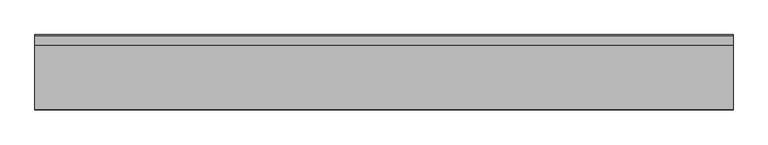
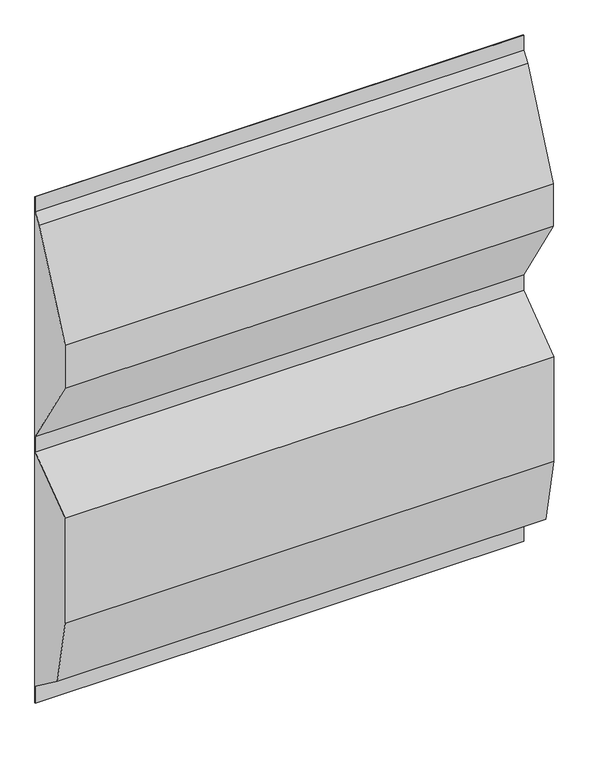
"""IFC4 building model written with IfcOpenShell, lengths in millimetres: proxy geometry, Generic Models 7:Generic Models 1:337419:Generic Models 1:337419 : Generic Models 7:Generic Models 1:337419:8 : Generic Models 7:Generic Models 1:337419:Generic Models 1:337419 : Generic Models 7:Generic Models 1:337419:301336."""

from ifc_helpers import new_model, si_unit, frame, origin, place, context, project, spatial, polyline, outline, extrude, source, transform, mapped, element, save


def generic_models_5b9c7308(model_context):
    return source(origin(), model_context, "Body", "SweptSolid", [
        extrude(outline(polyline([(-536554.1163358, 90.6507615), (-536554.1163358, 11.283024), (-536557.2913358, 11.283024), (-536557.2913358, 97.8057956), (-536744.5118881, 238.8866011), (-536811.2913841, 577.8151499), (-536811.2913841, 1117.5648692), (-536557.2913358, 1306.0805705), (-536557.2913358, 1385.45553), (-536808.6805724, 1787.7624055), (-536808.6805724, 2009.189072), (-536591.6998949, 2496.535653), (-536557.2913358, 2544.3305705), (-536557.2913358, 2620.927405), (-536554.1163358, 2620.927405), (-536554.1163358, 90.6507615)])), frame((593801.5867242, 0.0, 0.0), z_axis=(1.0, 0.0, 0.0), x_axis=(0.0, 1.0, 0.0)), (0.0, 0.0, 1.0), 2381.25),
    ])


if __name__ == "__main__":
    model = new_model("IFC4")
    model_context = context("Model", 3, world=origin())
    ifc_project = project(units=[si_unit("LENGTHUNIT", "METRE", prefix="MILLI")], contexts=[model_context])
    site = spatial("IfcSite", under=ifc_project)
    building = spatial("IfcBuilding", under=site)
    placement = place(None, origin())
    generic_models_shape = generic_models_5b9c7308(model_context)
    element("IfcBuildingElementProxy", 1, Name="Generic Models 7:Generic Models 1:337419:Generic Models 1:337419 : Generic Models 7:Generic Models 1:337419:8 : Generic Models 7:Generic Models 1:337419:Generic Models 1:337419 : Generic Models 7:Generic Models 1:337419:301336", ObjectType="Generic Models 7:Generic Models 1:337419:Generic Models 1:337419 : Generic Models 7:Generic Models 1:337419:8 : Generic Models 7:Generic Models 1:337419:Generic Models 1:337419 : Generic Models 7:Generic Models 1:337419:301336", at=placement, inside=building, context=model_context, shape_type="MappedRepresentation", body=[
        mapped(generic_models_shape, transform((0.0, 0.0, 0.0), x_axis=(1.0, 0.0, 0.0), y_axis=(0.0, 1.0, 0.0), z_axis=(0.0, 0.0, 1.0))),
    ])
    save(model, "model.ifc")

# Revit data of these elements
# Type "Generic Models 7:Generic Models 1:337419:Generic Models 1:337419 : Generic Models 7:Generic Models 1:337419:8 : Generic Models 7:Generic Models 1:337419:Generic Models 1:337419 : Generic Models 7:Generic Models 1:337419:301336"
#   NameOverride = "Generic Models 7:Generic Models 1:337419:Generic Models 1:337419 : Generic Models 7:Generic Models 1:337419:301336"
#   ObjectTypeOverride = "Generic Models 1:337419 : Generic Models 7:Generic Models 1:337419"
#   Reference = "Generic Models 1"
#   Tag = "301336"
# Element 1 (IfcBuildingElementProxy, "Generic Models 7:Generic Models 1:337419:Generic Models 1:337419 : Generic Models 7:Generic Models 1:337419:8 : Generic Models 7:Generic Models 1:337419:Generic Models 1:337419 : Generic Models 7:Generic Models 1:337419:301336")
#   Materials on its faces: "CLASS A FIBERGLASS INSULATION WITH DURABLE VAPOR BARRIER (WHITE) LINE"
# Materials
#   "CLASS A FIBERGLASS INSULATION WITH DURABLE VAPOR BARRIER (WHITE) LINE": class "Unassigned", colour RGB 187 139 199, transparency 0, Cost = 0
